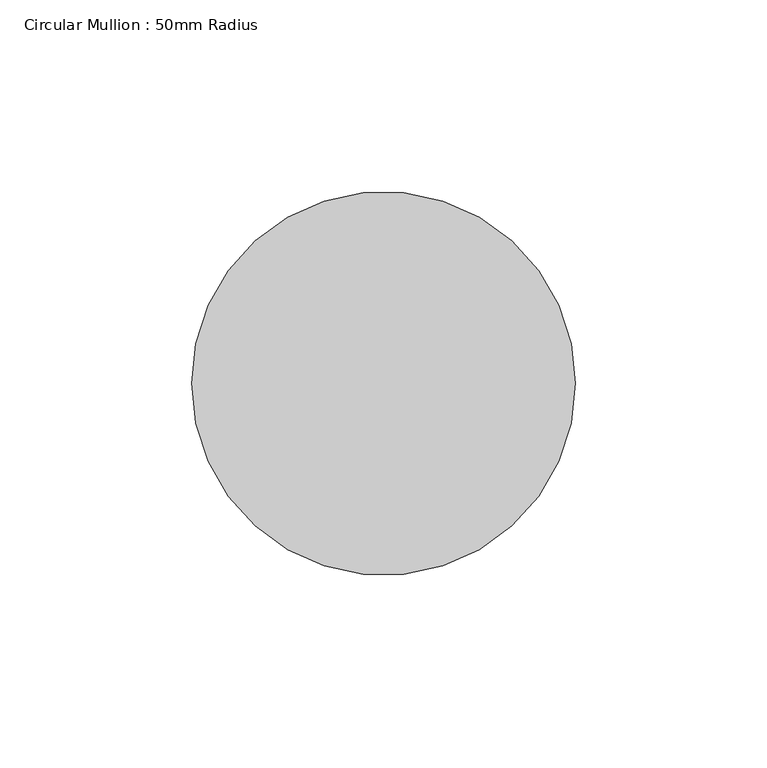
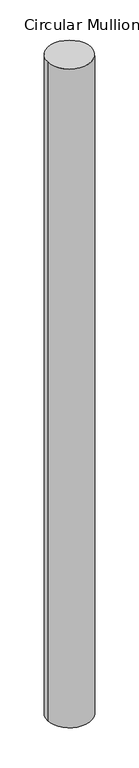
"""IFC4 building model written with IfcOpenShell, lengths in millimetres: member geometry, Circular Mullion : 50mm Radius."""

from ifc_helpers import new_model, si_unit, point, frame, origin, origin_2d, place, context, project, spatial, circle_curve, trimmed, segment, composite_curve, outline, extrude, source, transform, mapped, element, save


def circular_mullion_50mm_radius_e5d04943(model_context):
    return source(origin(), model_context, "Body", "SweptSolid", [
        extrude(outline(composite_curve([segment(trimmed(circle_curve(origin_2d(), 50.0), [point((50.0, 0.0))], [point((-50.0, 0.0))], False, "CARTESIAN"), True, "CONTINUOUS"), segment(trimmed(circle_curve(origin_2d(), 50.0), [point((-50.0, 0.0))], [point((50.0, 0.0))], False, "CARTESIAN"), True, "CONTINUOUS")], self_intersect=False)), frame((0.0, 0.0, -1593.7696074), z_axis=(0.0, 0.0, 1.0), x_axis=(1.0, 0.0, 0.0)), (0.0, 0.0, 1.0), 1593.7696074),
    ])


if __name__ == "__main__":
    model = new_model("IFC4")
    model_context = context("Model", 3, world=origin())
    ifc_project = project(units=[si_unit("LENGTHUNIT", "METRE", prefix="MILLI")], contexts=[model_context])
    site = spatial("IfcSite", under=ifc_project)
    building = spatial("IfcBuilding", under=site)
    placement = place(None, origin())
    circular_mullion_50mm_radius_shape = circular_mullion_50mm_radius_e5d04943(model_context)
    element("IfcMember", 1, ObjectType="Circular Mullion : 50mm Radius", at=placement, inside=building, context=model_context, shape_type="MappedRepresentation", body=[
        mapped(circular_mullion_50mm_radius_shape, transform((0.0, 0.0, 0.0), x_axis=(1.0, 0.0, 0.0), y_axis=(0.0, 1.0, 0.0), z_axis=(0.0, 0.0, 1.0))),
    ])
    save(model, "model.ifc")

# Revit data of these elements
# Type "Circular Mullion : 50mm Radius"
#   built-in parameter 1007350 = 0.164042 (stored number, unit not read)
# Element 1 (IfcMember, "Circular Mullion : 50mm Radius")
#   Materials on its faces: "Aluminium"
# Materials
#   "Aluminium": class "Metal", colour RGB 247 247 247, transparency 0, Description = "Aluminium 6061", Cost = 0
